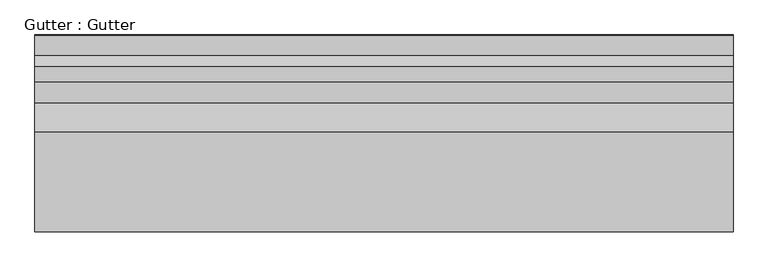
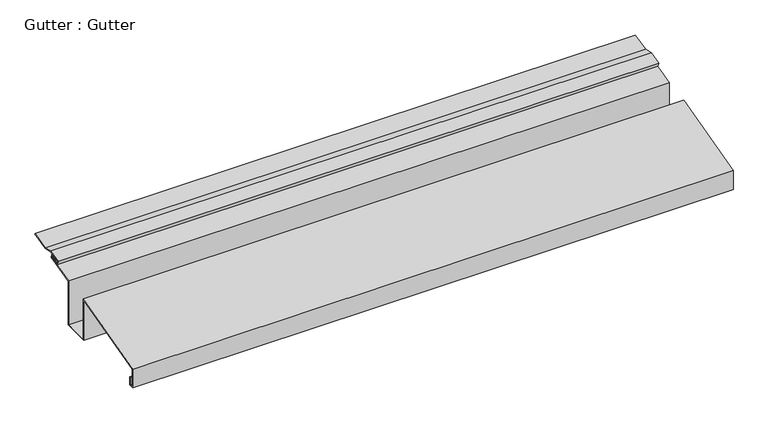
"""IFC4 building model written with IfcOpenShell, lengths in millimetres: proxy geometry, Gutter : Gutter."""

from ifc_helpers import new_model, si_unit, frame, origin, place, context, project, spatial, polyline, outline, extrude, source, transform, mapped, element, save


def gutter_gutter_0cab9b29(model_context):
    return source(origin(), model_context, "Body", "SweptSolid", [
        extrude(outline(polyline([(-5188.0399366, 42845.4152198), (-5191.2296164, 42857.7081422), (-5148.076519, 42868.8615907), (-5116.0538772, 42860.7718241), (-5057.619141, 42875.875), (-5056.9835337, 42873.4158124), (-5116.0466964, 42858.150212), (-5148.0693383, 42866.2399786), (-5188.1324915, 42855.8851642), (-5186.2186842, 42848.5094129), (-5160.7922022, 42855.0811997), (-5160.156595, 42852.6220122), (-5188.0399366, 42845.4152198)])), frame((12382.7678845, 0.0, 0.0), z_axis=(1.0, 0.0, 0.0), x_axis=(0.0, 1.0, 0.0)), (0.0, 0.0, 1.0), 2000.25),
        extrude(outline(polyline([(-5155.0377891, 42861.5014303), (-5151.8597529, 42849.2054925), (-5249.134388, 42824.0636673), (-5249.134388, 42669.601563), (-5339.089844, 42669.601563), (-5339.089844, 42811.566406), (-5618.8287201, 42737.492187), (-5618.8287201, 42675.5879789), (-5606.1287201, 42675.5879789), (-5606.1287201, 42700.9879789), (-5603.5887201, 42700.9879789), (-5603.5887201, 42673.0479789), (-5621.3687201, 42673.0479789), (-5621.3687201, 42739.4471419), (-5336.549844, 42814.8665333), (-5336.549844, 42672.141563), (-5251.674388, 42672.141563), (-5251.674388, 42826.0306412), (-5154.9545477, 42851.0290728), (-5156.8613694, 42858.4066355), (-5177.4570652, 42853.0834248), (-5178.0926724, 42855.5426123), (-5155.0377891, 42861.5014303)])), frame((12382.7678845, 0.0, 0.0), z_axis=(1.0, 0.0, 0.0), x_axis=(0.0, 1.0, 0.0)), (0.0, 0.0, 1.0), 2000.25),
    ])


if __name__ == "__main__":
    model = new_model("IFC4")
    model_context = context("Model", 3, world=origin())
    ifc_project = project(units=[si_unit("LENGTHUNIT", "METRE", prefix="MILLI")], contexts=[model_context])
    site = spatial("IfcSite", under=ifc_project)
    building = spatial("IfcBuilding", under=site)
    placement = place(None, origin())
    gutter_gutter_shape = gutter_gutter_0cab9b29(model_context)
    element("IfcBuildingElementProxy", 1, Name="Gutter : Gutter", ObjectType="Gutter : Gutter", at=placement, inside=building, context=model_context, shape_type="MappedRepresentation", body=[
        mapped(gutter_gutter_shape, transform((0.0, 0.0, 0.0), x_axis=(1.0, 0.0, 0.0), y_axis=(0.0, 1.0, 0.0), z_axis=(0.0, 0.0, 1.0))),
    ])
    save(model, "model.ifc")

# Revit data of these elements
# Type "Gutter : Gutter"
#   NameOverride = "Gutter"
# Element 1 (IfcBuildingElementProxy, "Gutter : Gutter")
#   Materials on its faces: "CONT. SEAMLESS 16 GA COPPER BRAKE METAL GUTTER"
# Materials
#   "CONT. SEAMLESS 16 GA COPPER BRAKE METAL GUTTER": class "Unassigned", colour RGB 128 128 128, transparency 0
